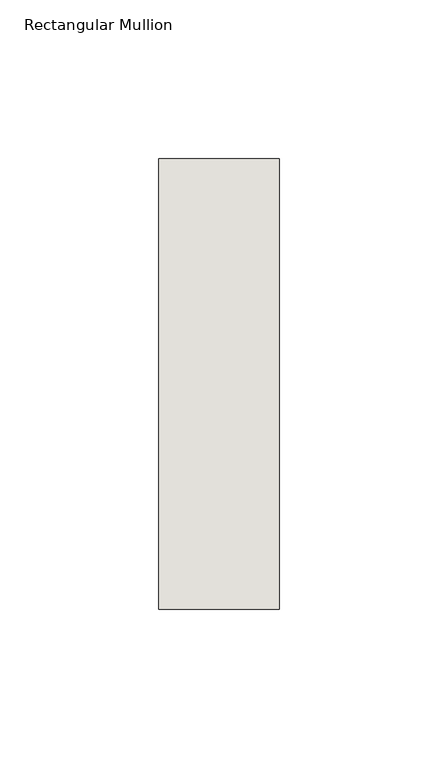
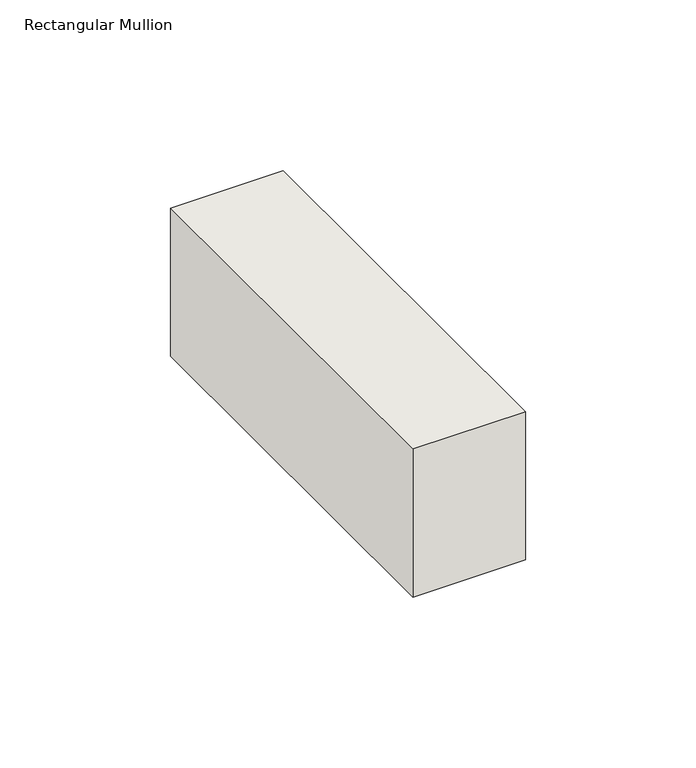
"""IFC4 building model written with IfcOpenShell, lengths in millimetres: wall geometry, Rectangular Mullion : NLRS_21_CWM_hsb-regel 38x142_gen_rsf."""

from ifc_helpers import new_model, si_unit, frame, origin, place, context, project, spatial, polyline, outline, extrude, source, transform, mapped, element, save


def rectangular_mullion_03633001(model_context):
    return source(origin(), model_context, "Body", "SweptSolid", [
        extrude(outline(polyline([(0.0, -71.0), (-38.0, -71.0), (-38.0, 71.0), (0.0, 71.0), (0.0, -71.0)])), frame((0.0, 0.0, -52.9999997), z_axis=(0.0, 0.0, 1.0), x_axis=(1.0, 0.0, 0.0)), (0.0, 0.0, 1.0), 52.9999997),
    ])


if __name__ == "__main__":
    model = new_model("IFC4")
    model_context = context("Model", 3, world=origin())
    ifc_project = project(units=[si_unit("LENGTHUNIT", "METRE", prefix="MILLI")], contexts=[model_context])
    site = spatial("IfcSite", under=ifc_project)
    building = spatial("IfcBuilding", under=site)
    placement = place(None, origin())
    rectangular_mullion_shape = rectangular_mullion_03633001(model_context)
    element("IfcWall", 1, ObjectType="Rectangular Mullion : NLRS_21_CWM_hsb-regel 38x142_gen_rsf", at=placement, inside=building, context=model_context, shape_type="MappedRepresentation", body=[
        mapped(rectangular_mullion_shape, transform((0.0, 0.0, 0.0), x_axis=(1.0, 0.0, 0.0), y_axis=(0.0, 1.0, 0.0), z_axis=(0.0, 0.0, 1.0))),
    ])
    save(model, "model.ifc")

# Revit data of these elements
# Type "Rectangular Mullion : NLRS_21_CWM_hsb-regel 38x142_gen_rsf"
#   Type IfcGUID = "07M7mRoiH1CR8m_RSKIwpF"
#   Assembly Code = "21.10"
#   IfcExportAs = "IfcWall"
#   built-in parameter 1007322 = 0.465879 (stored number, unit not read)
#   built-in parameter 1007321 = 0.062336 (stored number, unit not read)
#   built-in parameter 1007320 = 0.062336 (stored number, unit not read)
# Element 1 (IfcWall, "Rectangular Mullion : NLRS_21_CWM_hsb-regel 38x142_gen_rsf")
#   Materials on its faces: "NLRS_i2_hout naaldhout vuren_gen_rsf"
# Materials
#   "NLRS_i2_hout naaldhout vuren_gen_rsf": class "I - Hout", colour RGB 234 199 147, transparency 0, Keynote = "i2", Manufacturer = "Revit Standards Foundation", URL = "www.revitstandards.org", Description = "hout vuren", Cost = 0
